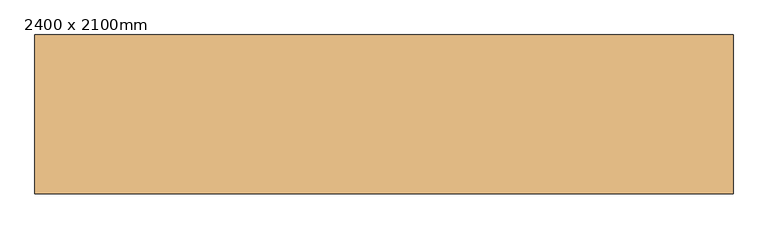
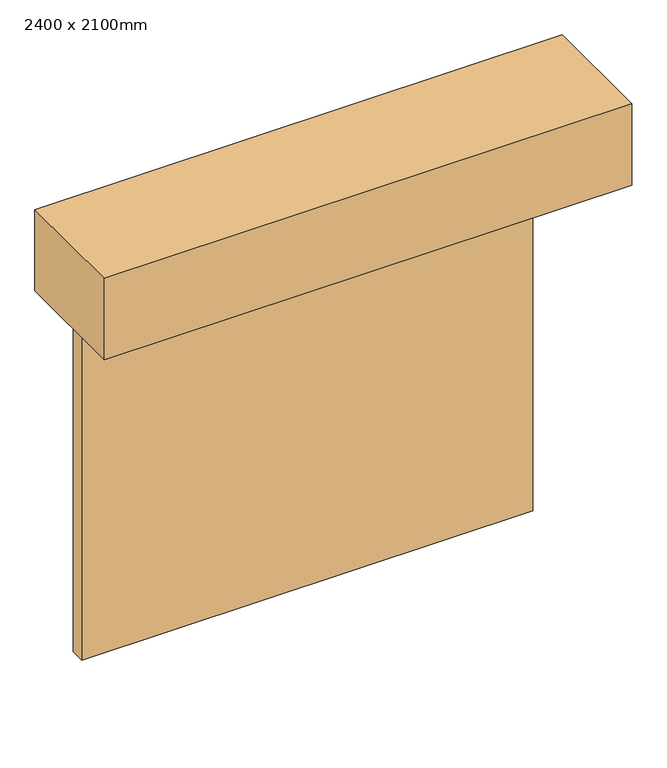
"""IFC4 building model written with IfcOpenShell, lengths in millimetres: door geometry, 滑升门 : 2400 x 2100mm."""

import ifcopenshell
import ifcopenshell.guid

model = None  # the IFC model being written
_history = None  # IfcOwnerHistory: only IFC2X3 demands one
_inside = {}  # id of a spatial element -> (the spatial element, [elements in it])
_under = {}  # id of a project, library or spatial element -> (it, [spatial elements below it])
_declared = {}  # id of a project -> (the project, [libraries it declares])
_typed = {}  # id of a type object -> (the type object, [elements of that type])
_made_of = {}  # id of a material, layer set ... -> (it, [elements and type objects made of it])


def new_model(schema):
    """Start an empty IFC model of exactly this schema.

    Asked for "IFC4X3", IfcOpenShell would pick the latest addendum, in which some entities
    have other attributes; the version numbers below select the first issue.
    IFC2X3 requires an IfcOwnerHistory on every rooted entity: one is made here for all.
    """
    global model, _history
    if schema == "IFC4X3":
        model = ifcopenshell.file(schema_version=(4, 3, 0, 0))
    else:
        model = ifcopenshell.file(schema=schema)
    _inside.clear()
    _under.clear()
    _declared.clear()
    _typed.clear()
    _made_of.clear()
    _history = None
    if model.schema == "IFC2X3":
        org = make("IfcOrganization", Name="unknown")
        user = make(
            "IfcPersonAndOrganization",
            ThePerson=make("IfcPerson", FamilyName="unknown"),
            TheOrganization=org,
        )
        app = make(
            "IfcApplication",
            ApplicationDeveloper=org,
            Version="unknown",
            ApplicationFullName="unknown",
            ApplicationIdentifier="unknown",
        )
        _history = make(
            "IfcOwnerHistory",
            OwningUser=user,
            OwningApplication=app,
            ChangeAction="ADDED",
            CreationDate=0,
        )
    return model


def make(cls, **values):
    """One entity of the class cls with the attributes given. An attribute that is None is left unset."""
    return model.create_entity(
        cls, **{name: value for name, value in values.items() if value is not None}
    )


def rooted(cls, **values):
    """An entity with a GlobalId (a new one), such as an element, a storey or a relation."""
    return make(cls, GlobalId=ifcopenshell.guid.new(), OwnerHistory=_history, **values)


def si_unit(unit_type, name, prefix=None):
    """IfcSIUnit, for example si_unit("LENGTHUNIT", "METRE", prefix="MILLI")."""
    return make("IfcSIUnit", UnitType=unit_type, Prefix=prefix, Name=name)


def assignment(units):
    """IfcUnitAssignment: the units of a project."""
    return None if units is None else make("IfcUnitAssignment", Units=units)


def point(xyz):
    """IfcCartesianPoint."""
    return None if xyz is None else make("IfcCartesianPoint", Coordinates=xyz)


def direction(xyz):
    """IfcDirection."""
    return None if xyz is None else make("IfcDirection", DirectionRatios=xyz)


def frame(location, z_axis=None, x_axis=None):
    """IfcAxis2Placement3D, a coordinate frame: its origin and axes. An axis left out is left unset."""
    return make(
        "IfcAxis2Placement3D",
        Location=point(location),
        Axis=direction(z_axis),
        RefDirection=direction(x_axis),
    )


def origin():
    """The frame at (0, 0, 0) with its axes left unset."""
    return frame((0.0, 0.0, 0.0))


def origin_with_axes():
    """The frame at (0, 0, 0) with the z axis (0, 0, 1) and the x axis (1, 0, 0) written out."""
    return frame((0.0, 0.0, 0.0), z_axis=(0.0, 0.0, 1.0), x_axis=(1.0, 0.0, 0.0))


def place(relative_to, where):
    """IfcLocalPlacement: puts the frame where relative to a parent placement (None: the world)."""
    return make(
        "IfcLocalPlacement", PlacementRelTo=relative_to, RelativePlacement=where
    )


def context(
    kind, dimensions, precision=None, world=None, true_north=None, identifier=None
):
    """IfcGeometricRepresentationContext, for example the 3D "Model" context."""
    return make(
        "IfcGeometricRepresentationContext",
        ContextIdentifier=identifier,
        ContextType=kind,
        CoordinateSpaceDimension=dimensions,
        Precision=precision,
        WorldCoordinateSystem=world,
        TrueNorth=true_north,
    )


def project(units=None, contexts=None):
    """IfcProject with its units and contexts."""
    return rooted(
        "IfcProject",
        Name="project",
        RepresentationContexts=contexts,
        UnitsInContext=assignment(units),
    )


def spatial(cls, under=None, at=None, **own):
    """A site, building, storey or space (cls), placed at a placement, below another one or the project."""
    s = rooted(cls, ObjectPlacement=at, **own)
    if under is not None:
        _under.setdefault(under.id(), (under, []))[1].append(s)
    return s


def polyline(points):
    """IfcPolyline through the points."""
    return make("IfcPolyline", Points=[point(p) for p in points])


def outline(outer, holes=None, kind="AREA"):
    """IfcArbitraryClosedProfileDef: a profile drawn as a closed curve; with holes, ...WithVoids."""
    if holes is None:
        return make("IfcArbitraryClosedProfileDef", ProfileType=kind, OuterCurve=outer)
    return make(
        "IfcArbitraryProfileDefWithVoids",
        ProfileType=kind,
        OuterCurve=outer,
        InnerCurves=holes,
    )


def extrude(swept, where, along, depth):
    """IfcExtrudedAreaSolid: the profile swept, set in the frame where, extruded along a direction by depth."""
    return make(
        "IfcExtrudedAreaSolid",
        SweptArea=swept,
        Position=where,
        ExtrudedDirection=direction(along),
        Depth=depth,
    )


def shape(context_of_items, identifier, shape_type, items):
    """IfcShapeRepresentation: the items that make up one representation, for example the "Body"."""
    return make(
        "IfcShapeRepresentation",
        ContextOfItems=context_of_items,
        RepresentationIdentifier=identifier,
        RepresentationType=shape_type,
        Items=items,
    )


def source(mapping_origin, context_of_items, identifier, shape_type, items):
    """IfcRepresentationMap: a shape defined once, which mapped items show again and again."""
    return make(
        "IfcRepresentationMap",
        MappingOrigin=mapping_origin,
        MappedRepresentation=shape(context_of_items, identifier, shape_type, items),
    )


def transform(
    local_origin,
    x_axis=None,
    y_axis=None,
    z_axis=None,
    scale=None,
    scale2=None,
    scale3=None,
    uniform=True,
):
    """IfcCartesianTransformationOperator3D, or its non-uniform kind. x_axis, y_axis, z_axis: its Axis1, 2, 3."""
    if uniform:
        return make(
            "IfcCartesianTransformationOperator3D",
            Axis1=direction(x_axis),
            Axis2=direction(y_axis),
            LocalOrigin=point(local_origin),
            Scale=scale,
            Axis3=direction(z_axis),
        )
    return make(
        "IfcCartesianTransformationOperator3DnonUniform",
        Axis1=direction(x_axis),
        Axis2=direction(y_axis),
        LocalOrigin=point(local_origin),
        Scale=scale,
        Axis3=direction(z_axis),
        Scale2=scale2,
        Scale3=scale3,
    )


def mapped(mapping_source, mapping_target):
    """IfcMappedItem: shows the shape of a source again, moved by a transform."""
    return make(
        "IfcMappedItem", MappingSource=mapping_source, MappingTarget=mapping_target
    )


def made_of(thing, what):
    """Note that an element or type object is made of a material, layer set ...; save() writes the relation."""
    if what is not None:
        _made_of.setdefault(what.id(), (what, []))[1].append(thing)
    return thing


def element(
    cls,
    number,
    at=None,
    inside=None,
    cuts=None,
    type_object=None,
    material=None,
    context=None,
    identifier="Body",
    shape_type=None,
    held_by="IfcProductDefinitionShape",
    body=None,
    shapes=None,
    **own,
):
    """One element of the class cls, such as IfcWall. Its Tag is "e" and its number.

    at: its placement. inside: the storey or other place that contains it. cuts: it is an
    opening in that element (IfcRelVoidsElement). A single representation is given by context,
    identifier, shape_type and body (its items); several are given by shapes. held_by: the class
    of the entity that holds the representations. save() writes the other relations.
    """
    e = rooted(cls, Tag="e%d" % number, ObjectPlacement=at, **own)
    if body is not None:
        shapes = [shape(context, identifier, shape_type, body)]
    if shapes is not None:
        e.Representation = make(held_by, Representations=shapes)
    if inside is not None:
        _inside.setdefault(inside.id(), (inside, []))[1].append(e)
    if cuts is not None:
        rooted(
            "IfcRelVoidsElement", RelatingBuildingElement=cuts, RelatedOpeningElement=e
        )
    if type_object is not None:
        _typed.setdefault(type_object.id(), (type_object, []))[1].append(e)
    return made_of(e, material)


def aggregate(whole, parts):
    """IfcRelAggregates: a whole, such as a stair, and the parts it consists of."""
    return rooted("IfcRelAggregates", RelatingObject=whole, RelatedObjects=parts)


def save(model, path):
    """Write the relations noted so far, then the file.

    IfcRelAggregates (storeys below a building ...), IfcRelContainedInSpatialStructure (elements
    in a storey), IfcRelDefinesByType, IfcRelAssociatesMaterial and IfcRelDeclares: one each for
    every whole, place, type object, material and project.
    """
    for whole, parts in _under.values():
        aggregate(whole, parts)
    for where, things in _inside.values():
        rooted(
            "IfcRelContainedInSpatialStructure",
            RelatedElements=things,
            RelatingStructure=where,
        )
    for kind, things in _typed.values():
        rooted("IfcRelDefinesByType", RelatedObjects=things, RelatingType=kind)
    for what, things in _made_of.values():
        rooted("IfcRelAssociatesMaterial", RelatedObjects=things, RelatingMaterial=what)
    for by, libraries in _declared.values():
        rooted("IfcRelDeclares", RelatingContext=by, RelatedDefinitions=libraries)
    model.write(path)


def door_2400_x_2100mm_76126092(model_context):
    return source(origin(), model_context, "Body", "SweptSolid", [
        extrude(outline(polyline([(1200.0, -120.0), (1200.0, -200.0), (-1200.0, -200.0), (-1200.0, -120.0), (1200.0, -120.0)])), origin_with_axes(), (0.0, 0.0, 1.0), 2100.0),
        extrude(outline(polyline([(1403.2, -758.8), (-1403.2, -758.8), (-1403.2, -120.0), (1403.2, -120.0), (1403.2, -758.8)])), frame((0.0, 0.0, 2100.0), z_axis=(0.0, 0.0, 1.0), x_axis=(1.0, 0.0, 0.0)), (0.0, 0.0, 1.0), 457.2),
    ])


if __name__ == "__main__":
    model = new_model("IFC4")
    model_context = context("Model", 3, world=origin())
    ifc_project = project(units=[si_unit("LENGTHUNIT", "METRE", prefix="MILLI")], contexts=[model_context])
    site = spatial("IfcSite", under=ifc_project)
    building = spatial("IfcBuilding", under=site)
    placement = place(None, origin())
    door_2400_x_2100mm_shape = door_2400_x_2100mm_76126092(model_context)
    element("IfcDoor", 1, ObjectType="滑升门 : 2400 x 2100mm", at=placement, inside=building, context=model_context, shape_type="MappedRepresentation", body=[
        mapped(door_2400_x_2100mm_shape, transform((0.0, 0.0, 0.0), x_axis=(1.0, 0.0, 0.0), y_axis=(0.0, 1.0, 0.0), z_axis=(0.0, 0.0, 1.0))),
    ])
    save(model, "model.ifc")

# Revit data of these elements
# Type "滑升门 : 2400 x 2100mm"
#   Type Mark = "M837"
#   Construction Type Id = "MDOOR"
#   Analytic Construction = "金属"
#   Thickness = 80 mm
#   Rough Width = 2400 mm
#   Rough Height = 2100 mm
#   Height = 2100 mm
#   Width = 2400 mm
#   Heat Transfer Coefficient (U) = 3.7021 W/(m²·K)
#   卷帘盒可见性 [instance default] = yes
#   Function = 1
#   卷帘箱材质 = none
#   门嵌板材质 = none
#   Visual Light Transmittance = 0
#   Solar Heat Gain Coefficient = 0
#   Wall Closure = (empty or 0)
